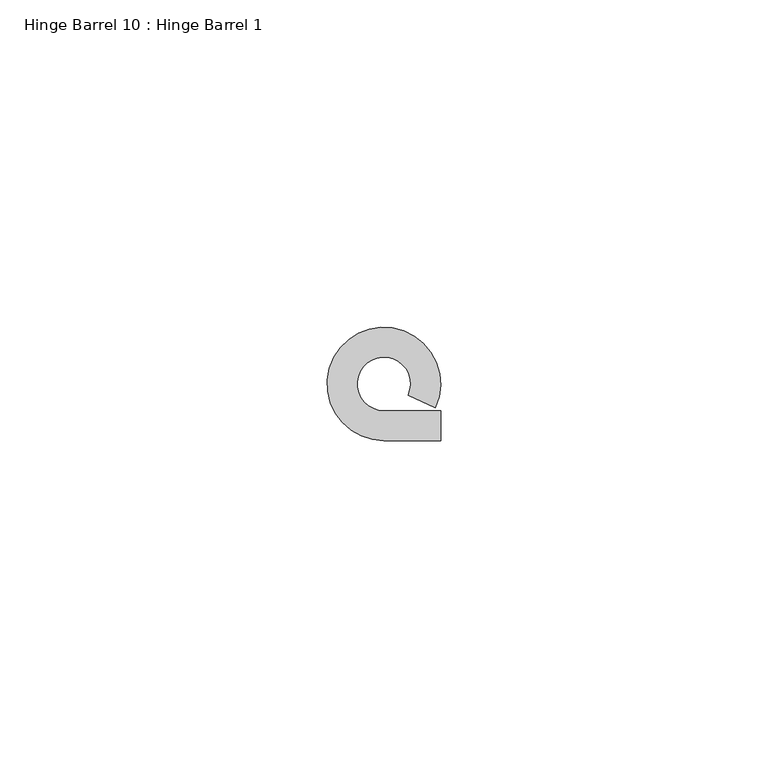
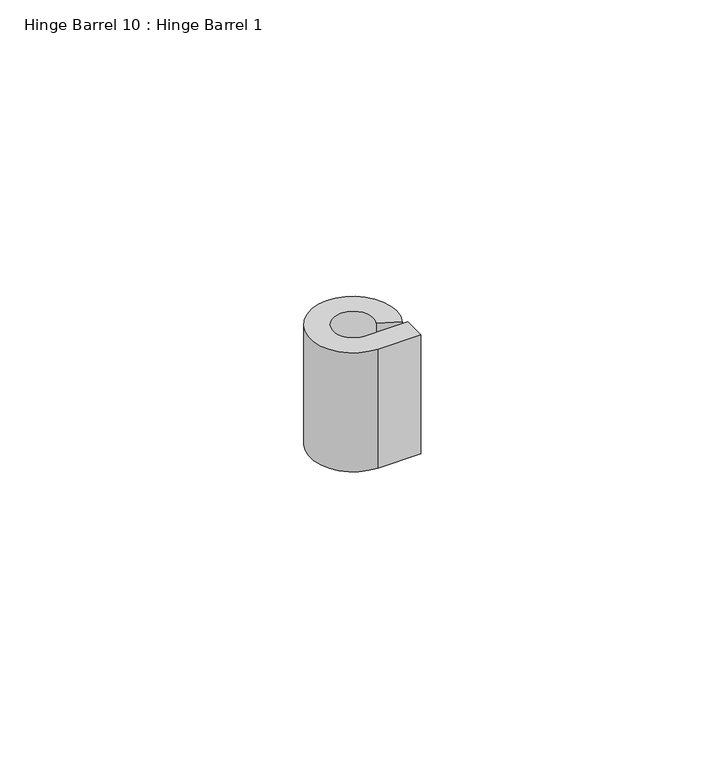
"""IFC4 building model written with IfcOpenShell, lengths in millimetres: proxy geometry, Hinge Barrel 10 : Hinge Barrel 1."""

import ifcopenshell
import ifcopenshell.guid

model = None  # the IFC model being written
_history = None  # IfcOwnerHistory: only IFC2X3 demands one
_inside = {}  # id of a spatial element -> (the spatial element, [elements in it])
_under = {}  # id of a project, library or spatial element -> (it, [spatial elements below it])
_declared = {}  # id of a project -> (the project, [libraries it declares])
_typed = {}  # id of a type object -> (the type object, [elements of that type])
_made_of = {}  # id of a material, layer set ... -> (it, [elements and type objects made of it])


def new_model(schema):
    """Start an empty IFC model of exactly this schema.

    Asked for "IFC4X3", IfcOpenShell would pick the latest addendum, in which some entities
    have other attributes; the version numbers below select the first issue.
    IFC2X3 requires an IfcOwnerHistory on every rooted entity: one is made here for all.
    """
    global model, _history
    if schema == "IFC4X3":
        model = ifcopenshell.file(schema_version=(4, 3, 0, 0))
    else:
        model = ifcopenshell.file(schema=schema)
    _inside.clear()
    _under.clear()
    _declared.clear()
    _typed.clear()
    _made_of.clear()
    _history = None
    if model.schema == "IFC2X3":
        org = make("IfcOrganization", Name="unknown")
        user = make(
            "IfcPersonAndOrganization",
            ThePerson=make("IfcPerson", FamilyName="unknown"),
            TheOrganization=org,
        )
        app = make(
            "IfcApplication",
            ApplicationDeveloper=org,
            Version="unknown",
            ApplicationFullName="unknown",
            ApplicationIdentifier="unknown",
        )
        _history = make(
            "IfcOwnerHistory",
            OwningUser=user,
            OwningApplication=app,
            ChangeAction="ADDED",
            CreationDate=0,
        )
    return model


def make(cls, **values):
    """One entity of the class cls with the attributes given. An attribute that is None is left unset."""
    return model.create_entity(
        cls, **{name: value for name, value in values.items() if value is not None}
    )


def rooted(cls, **values):
    """An entity with a GlobalId (a new one), such as an element, a storey or a relation."""
    return make(cls, GlobalId=ifcopenshell.guid.new(), OwnerHistory=_history, **values)


def si_unit(unit_type, name, prefix=None):
    """IfcSIUnit, for example si_unit("LENGTHUNIT", "METRE", prefix="MILLI")."""
    return make("IfcSIUnit", UnitType=unit_type, Prefix=prefix, Name=name)


def assignment(units):
    """IfcUnitAssignment: the units of a project."""
    return None if units is None else make("IfcUnitAssignment", Units=units)


def point(xyz):
    """IfcCartesianPoint."""
    return None if xyz is None else make("IfcCartesianPoint", Coordinates=xyz)


def direction(xyz):
    """IfcDirection."""
    return None if xyz is None else make("IfcDirection", DirectionRatios=xyz)


def frame(location, z_axis=None, x_axis=None):
    """IfcAxis2Placement3D, a coordinate frame: its origin and axes. An axis left out is left unset."""
    return make(
        "IfcAxis2Placement3D",
        Location=point(location),
        Axis=direction(z_axis),
        RefDirection=direction(x_axis),
    )


def frame_2d(location, x_axis=None):
    """IfcAxis2Placement2D, a coordinate frame in the plane: its origin and x axis."""
    return make(
        "IfcAxis2Placement2D", Location=point(location), RefDirection=direction(x_axis)
    )


def origin():
    """The frame at (0, 0, 0) with its axes left unset."""
    return frame((0.0, 0.0, 0.0))


def place(relative_to, where):
    """IfcLocalPlacement: puts the frame where relative to a parent placement (None: the world)."""
    return make(
        "IfcLocalPlacement", PlacementRelTo=relative_to, RelativePlacement=where
    )


def context(
    kind, dimensions, precision=None, world=None, true_north=None, identifier=None
):
    """IfcGeometricRepresentationContext, for example the 3D "Model" context."""
    return make(
        "IfcGeometricRepresentationContext",
        ContextIdentifier=identifier,
        ContextType=kind,
        CoordinateSpaceDimension=dimensions,
        Precision=precision,
        WorldCoordinateSystem=world,
        TrueNorth=true_north,
    )


def project(units=None, contexts=None):
    """IfcProject with its units and contexts."""
    return rooted(
        "IfcProject",
        Name="project",
        RepresentationContexts=contexts,
        UnitsInContext=assignment(units),
    )


def spatial(cls, under=None, at=None, **own):
    """A site, building, storey or space (cls), placed at a placement, below another one or the project."""
    s = rooted(cls, ObjectPlacement=at, **own)
    if under is not None:
        _under.setdefault(under.id(), (under, []))[1].append(s)
    return s


def polyline(points):
    """IfcPolyline through the points."""
    return make("IfcPolyline", Points=[point(p) for p in points])


def circle_curve(where, radius):
    """IfcCircle in the frame where."""
    return make("IfcCircle", Position=where, Radius=radius)


def trimmed(basis, trim1, trim2, sense, master):
    """IfcTrimmedCurve: the piece of a basis curve between two trims."""
    return make(
        "IfcTrimmedCurve",
        BasisCurve=basis,
        Trim1=trim1,
        Trim2=trim2,
        SenseAgreement=sense,
        MasterRepresentation=master,
    )


def segment(curve, same_sense, transition):
    """IfcCompositeCurveSegment."""
    return make(
        "IfcCompositeCurveSegment",
        Transition=transition,
        SameSense=same_sense,
        ParentCurve=curve,
    )


def composite_curve(segments, self_intersect=None):
    """IfcCompositeCurve: segments joined end to end."""
    return make("IfcCompositeCurve", Segments=segments, SelfIntersect=self_intersect)


def outline(outer, holes=None, kind="AREA"):
    """IfcArbitraryClosedProfileDef: a profile drawn as a closed curve; with holes, ...WithVoids."""
    if holes is None:
        return make("IfcArbitraryClosedProfileDef", ProfileType=kind, OuterCurve=outer)
    return make(
        "IfcArbitraryProfileDefWithVoids",
        ProfileType=kind,
        OuterCurve=outer,
        InnerCurves=holes,
    )


def extrude(swept, where, along, depth):
    """IfcExtrudedAreaSolid: the profile swept, set in the frame where, extruded along a direction by depth."""
    return make(
        "IfcExtrudedAreaSolid",
        SweptArea=swept,
        Position=where,
        ExtrudedDirection=direction(along),
        Depth=depth,
    )


def shape(context_of_items, identifier, shape_type, items):
    """IfcShapeRepresentation: the items that make up one representation, for example the "Body"."""
    return make(
        "IfcShapeRepresentation",
        ContextOfItems=context_of_items,
        RepresentationIdentifier=identifier,
        RepresentationType=shape_type,
        Items=items,
    )


def source(mapping_origin, context_of_items, identifier, shape_type, items):
    """IfcRepresentationMap: a shape defined once, which mapped items show again and again."""
    return make(
        "IfcRepresentationMap",
        MappingOrigin=mapping_origin,
        MappedRepresentation=shape(context_of_items, identifier, shape_type, items),
    )


def transform(
    local_origin,
    x_axis=None,
    y_axis=None,
    z_axis=None,
    scale=None,
    scale2=None,
    scale3=None,
    uniform=True,
):
    """IfcCartesianTransformationOperator3D, or its non-uniform kind. x_axis, y_axis, z_axis: its Axis1, 2, 3."""
    if uniform:
        return make(
            "IfcCartesianTransformationOperator3D",
            Axis1=direction(x_axis),
            Axis2=direction(y_axis),
            LocalOrigin=point(local_origin),
            Scale=scale,
            Axis3=direction(z_axis),
        )
    return make(
        "IfcCartesianTransformationOperator3DnonUniform",
        Axis1=direction(x_axis),
        Axis2=direction(y_axis),
        LocalOrigin=point(local_origin),
        Scale=scale,
        Axis3=direction(z_axis),
        Scale2=scale2,
        Scale3=scale3,
    )


def mapped(mapping_source, mapping_target):
    """IfcMappedItem: shows the shape of a source again, moved by a transform."""
    return make(
        "IfcMappedItem", MappingSource=mapping_source, MappingTarget=mapping_target
    )


def made_of(thing, what):
    """Note that an element or type object is made of a material, layer set ...; save() writes the relation."""
    if what is not None:
        _made_of.setdefault(what.id(), (what, []))[1].append(thing)
    return thing


def element(
    cls,
    number,
    at=None,
    inside=None,
    cuts=None,
    type_object=None,
    material=None,
    context=None,
    identifier="Body",
    shape_type=None,
    held_by="IfcProductDefinitionShape",
    body=None,
    shapes=None,
    **own,
):
    """One element of the class cls, such as IfcWall. Its Tag is "e" and its number.

    at: its placement. inside: the storey or other place that contains it. cuts: it is an
    opening in that element (IfcRelVoidsElement). A single representation is given by context,
    identifier, shape_type and body (its items); several are given by shapes. held_by: the class
    of the entity that holds the representations. save() writes the other relations.
    """
    e = rooted(cls, Tag="e%d" % number, ObjectPlacement=at, **own)
    if body is not None:
        shapes = [shape(context, identifier, shape_type, body)]
    if shapes is not None:
        e.Representation = make(held_by, Representations=shapes)
    if inside is not None:
        _inside.setdefault(inside.id(), (inside, []))[1].append(e)
    if cuts is not None:
        rooted(
            "IfcRelVoidsElement", RelatingBuildingElement=cuts, RelatedOpeningElement=e
        )
    if type_object is not None:
        _typed.setdefault(type_object.id(), (type_object, []))[1].append(e)
    return made_of(e, material)


def aggregate(whole, parts):
    """IfcRelAggregates: a whole, such as a stair, and the parts it consists of."""
    return rooted("IfcRelAggregates", RelatingObject=whole, RelatedObjects=parts)


def save(model, path):
    """Write the relations noted so far, then the file.

    IfcRelAggregates (storeys below a building ...), IfcRelContainedInSpatialStructure (elements
    in a storey), IfcRelDefinesByType, IfcRelAssociatesMaterial and IfcRelDeclares: one each for
    every whole, place, type object, material and project.
    """
    for whole, parts in _under.values():
        aggregate(whole, parts)
    for where, things in _inside.values():
        rooted(
            "IfcRelContainedInSpatialStructure",
            RelatedElements=things,
            RelatingStructure=where,
        )
    for kind, things in _typed.values():
        rooted("IfcRelDefinesByType", RelatedObjects=things, RelatingType=kind)
    for what, things in _made_of.values():
        rooted("IfcRelAssociatesMaterial", RelatedObjects=things, RelatingMaterial=what)
    for by, libraries in _declared.values():
        rooted("IfcRelDeclares", RelatingContext=by, RelatedDefinitions=libraries)
    model.write(path)


def hinge_barrel_10_hinge_barrel_1_181395a2(model_context):
    return source(origin(), model_context, "Body", "SweptSolid", [
        extrude(outline(composite_curve([segment(polyline([(587323.2214739, -531780.6943841), (587327.7934739, -531780.6943841), (587327.7934739, -531785.2584466), (587319.1320739, -531785.2584466)]), True, "CONTINUOUS"), segment(trimmed(circle_curve(frame_2d((587319.1320739, -531776.6049841)), 8.6534625), [point((587319.1320739, -531785.2584466))], [point((587326.986084, -531780.2377433))], False, "CARTESIAN"), True, "CONTINUOUS"), segment(polyline([(587326.986084, -531780.2377433), (587322.8436736, -531778.321731)]), True, "CONTINUOUS"), segment(trimmed(circle_curve(frame_2d((587319.1320739, -531776.6049841)), 4.0894), [point((587322.8436736, -531778.321731))], [point((587319.1320739, -531780.6943841))], True, "CARTESIAN"), True, "CONTINUOUS"), segment(polyline([(587319.1320739, -531780.6943841), (587323.2214739, -531780.6943841)]), True, "CONTINUOUS")], self_intersect=False)), frame((0.0, 0.0, 2038.35), z_axis=(0.0, 0.0, 1.0), x_axis=(1.0, 0.0, 0.0)), (0.0, 0.0, 1.0), 25.4),
    ])


if __name__ == "__main__":
    model = new_model("IFC4")
    model_context = context("Model", 3, world=origin())
    ifc_project = project(units=[si_unit("LENGTHUNIT", "METRE", prefix="MILLI")], contexts=[model_context])
    site = spatial("IfcSite", under=ifc_project)
    building = spatial("IfcBuilding", under=site)
    placement = place(None, origin())
    hinge_barrel_10_hinge_barrel_1_shape = hinge_barrel_10_hinge_barrel_1_181395a2(model_context)
    element("IfcBuildingElementProxy", 1, Name="Hinge Barrel 10 : Hinge Barrel 1", ObjectType="Hinge Barrel 10 : Hinge Barrel 1", at=placement, inside=building, context=model_context, shape_type="MappedRepresentation", body=[
        mapped(hinge_barrel_10_hinge_barrel_1_shape, transform((0.0, 0.0, 0.0), x_axis=(1.0, 0.0, 0.0), y_axis=(0.0, 1.0, 0.0), z_axis=(0.0, 0.0, 1.0))),
    ])
    save(model, "model.ifc")

# Revit data of these elements
# Element 1 (IfcBuildingElementProxy, "Hinge Barrel 10 : Hinge Barrel 1")
#   Materials on its faces: "6\"X6\" WELD-ON STL BUTT HINGE"
# Materials
#   "6\"X6\" WELD-ON STL BUTT HINGE": class "Metal", colour RGB 189 187 185, transparency 0, Description = "Carbon steel", Cost = 0
